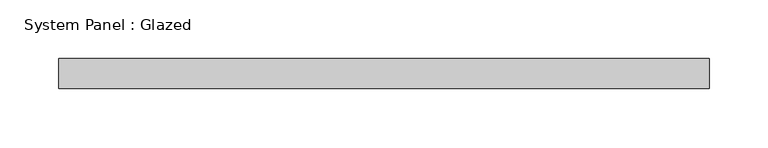
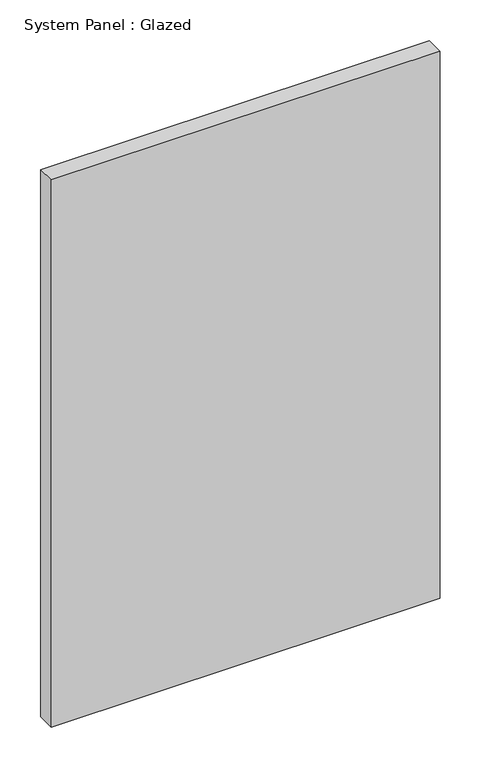
"""IFC4 building model written with IfcOpenShell, lengths in millimetres: plate geometry, System Panel : Glazed."""

from ifc_helpers import new_model, si_unit, origin, origin_with_axes, place, context, project, spatial, polyline, outline, extrude, source, transform, mapped, element, save


def system_panel_glazed_739d6e45(model_context):
    return source(origin(), model_context, "Body", "SweptSolid", [
        extrude(outline(polyline([(275.5179765, 19.05), (-275.5179765, 19.05), (-275.5179765, 44.45), (275.5179765, 44.45), (275.5179765, 19.05)])), origin_with_axes(), (0.0, 0.0, 1.0), 819.15),
    ])


if __name__ == "__main__":
    model = new_model("IFC4")
    model_context = context("Model", 3, world=origin())
    ifc_project = project(units=[si_unit("LENGTHUNIT", "METRE", prefix="MILLI")], contexts=[model_context])
    site = spatial("IfcSite", under=ifc_project)
    building = spatial("IfcBuilding", under=site)
    placement = place(None, origin())
    system_panel_glazed_shape = system_panel_glazed_739d6e45(model_context)
    element("IfcPlate", 1, ObjectType="System Panel : Glazed", at=placement, inside=building, context=model_context, shape_type="MappedRepresentation", body=[
        mapped(system_panel_glazed_shape, transform((0.0, 0.0, 0.0), x_axis=(1.0, 0.0, 0.0), y_axis=(0.0, 1.0, 0.0), z_axis=(0.0, 0.0, 1.0))),
    ])
    save(model, "model.ifc")

# Revit data of these elements
# Element 1 (IfcPlate, "System Panel : Glazed")
#   Materials on its faces: "Glass"
# Materials
#   "Glass": class "Glass", colour RGB 0 128 192, transparency 0.75
